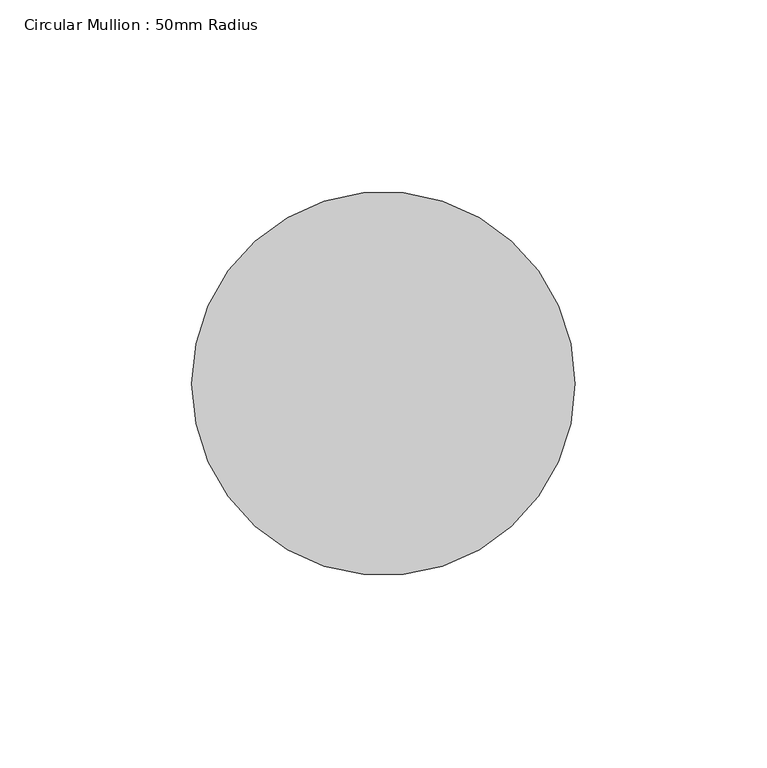
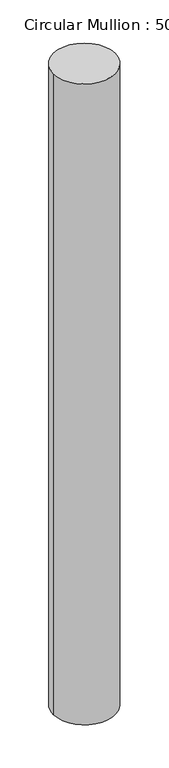
"""IFC4 building model written with IfcOpenShell, lengths in millimetres: member geometry, Circular Mullion : 50mm Radius."""

from ifc_helpers import new_model, si_unit, point, frame, origin, origin_2d, place, context, project, spatial, circle_curve, trimmed, segment, composite_curve, outline, extrude, source, transform, mapped, element, save


def circular_mullion_50mm_radius_dc684283(model_context):
    return source(origin(), model_context, "Body", "SweptSolid", [
        extrude(outline(composite_curve([segment(trimmed(circle_curve(origin_2d(), 50.0), [point((50.0, 0.0))], [point((-50.0, 0.0))], False, "CARTESIAN"), True, "CONTINUOUS"), segment(trimmed(circle_curve(origin_2d(), 50.0), [point((-50.0, 0.0))], [point((50.0, 0.0))], False, "CARTESIAN"), True, "CONTINUOUS")], self_intersect=False)), frame((0.0, 0.0, -1097.9709519), z_axis=(0.0, 0.0, 1.0), x_axis=(1.0, 0.0, 0.0)), (0.0, 0.0, 1.0), 1097.9709519),
    ])


if __name__ == "__main__":
    model = new_model("IFC4")
    model_context = context("Model", 3, world=origin())
    ifc_project = project(units=[si_unit("LENGTHUNIT", "METRE", prefix="MILLI")], contexts=[model_context])
    site = spatial("IfcSite", under=ifc_project)
    building = spatial("IfcBuilding", under=site)
    placement = place(None, origin())
    circular_mullion_50mm_radius_shape = circular_mullion_50mm_radius_dc684283(model_context)
    element("IfcMember", 1, ObjectType="Circular Mullion : 50mm Radius", at=placement, inside=building, context=model_context, shape_type="MappedRepresentation", body=[
        mapped(circular_mullion_50mm_radius_shape, transform((0.0, 0.0, 0.0), x_axis=(1.0, 0.0, 0.0), y_axis=(0.0, 1.0, 0.0), z_axis=(0.0, 0.0, 1.0))),
    ])
    save(model, "model.ifc")

# Revit data of these elements
# Type "Circular Mullion : 50mm Radius"
#   built-in parameter 1007350 = 0.164042 (stored number, unit not read)
# Element 1 (IfcMember, "Circular Mullion : 50mm Radius")
#   Materials on its faces: "Aluminium"
# Materials
#   "Aluminium": class "Metal", colour RGB 247 247 247, transparency 0, Description = "Aluminium 6061", Cost = 0
